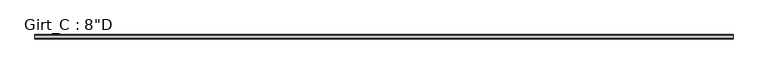
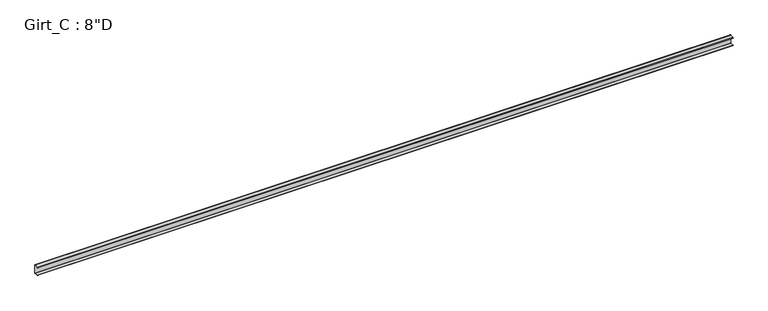
"""IFC4 building model written with IfcOpenShell, lengths in millimetres: beam geometry."""

from ifc_helpers import new_model, si_unit, point, frame, frame_2d, origin, place, context, project, spatial, polyline, circle_curve, trimmed, segment, composite_curve, outline, extrude, source, transform, mapped, element, save


def beam_ff75d66e(model_context):
    return source(origin(), model_context, "Body", "SweptSolid", [
        extrude(outline(composite_curve([segment(polyline([(-87.5109375, 101.6), (-3.3734375, 101.6)]), True, "CONTINUOUS"), segment(trimmed(circle_curve(frame_2d((-3.3734375, 96.8375)), 4.7625), [point((-3.3734375, 101.6))], [point((1.3890625, 96.8375))], False, "CARTESIAN"), True, "CONTINUOUS"), segment(polyline([(1.3890625, 96.8375), (1.3890625, -96.8375)]), True, "CONTINUOUS"), segment(trimmed(circle_curve(frame_2d((-3.3734375, -96.8375)), 4.7625), [point((1.3890625, -96.8375))], [point((-3.3734375, -101.6))], False, "CARTESIAN"), True, "CONTINUOUS"), segment(polyline([(-3.3734375, -101.6), (-87.5109375, -101.6), (-99.7792647, -86.979177), (-97.6510975, -85.1934327), (-86.2154765, -98.821875), (-3.2694106, -98.821875)]), True, "CONTINUOUS"), segment(trimmed(circle_curve(frame_2d((-3.3748024, -96.8389339)), 1.9857399), [point((-3.2694106, -98.821875))], [point((-1.3890625, -96.8389339))], True, "CARTESIAN"), True, "CONTINUOUS"), segment(polyline([(-1.3890625, -96.8389339), (-1.3890625, 96.8381931)]), True, "CONTINUOUS"), segment(trimmed(circle_curve(frame_2d((-3.3741066, 96.8381931)), 1.9850441), [point((-1.3890625, 96.8381931))], [point((-3.3005807, 98.821875))], True, "CARTESIAN"), True, "CONTINUOUS"), segment(polyline([(-3.3005807, 98.821875), (-86.2154765, 98.821875), (-97.6278742, 85.221109), (-99.7560415, 87.0068534), (-87.5109375, 101.6)]), True, "CONTINUOUS")], self_intersect=False)), frame((-7957.5904341, 0.0, 0.0), z_axis=(1.0, 0.0, 0.0), x_axis=(0.0, 1.0, 0.0)), (0.0, 0.0, 1.0), 15851.7537415),
    ])


if __name__ == "__main__":
    model = new_model("IFC4")
    model_context = context("Model", 3, world=origin())
    ifc_project = project(units=[si_unit("LENGTHUNIT", "METRE", prefix="MILLI")], contexts=[model_context])
    site = spatial("IfcSite", under=ifc_project)
    building = spatial("IfcBuilding", under=site)
    placement = place(None, origin())
    beam_shape = beam_ff75d66e(model_context)
    element("IfcBeam", 1, ObjectType="Girt_C : 8\"D", at=placement, inside=building, context=model_context, shape_type="MappedRepresentation", body=[
        mapped(beam_shape, transform((0.0, 0.0, 0.0), x_axis=(1.0, 0.0, 0.0), y_axis=(0.0, 1.0, 0.0), z_axis=(0.0, 0.0, 1.0))),
    ])
    save(model, "model.ifc")

# Revit data of these elements
# Type "Girt_C : 8\"D"
#   half leg = 0' - 1 3/4"
#   Web_Thickness = 0' - 0 7/64"
#   Length [instance default] = 10' - 0"
#   Leg_1 = 0' - 3 1/2"
#   Height = 0' - 8"
#   Structural Material [instance default] = none
# Element 1 (IfcBeam, "Girt_C : 8\"D")
#   Structural Material = GALVANIZED 'CEE' SECTION (8.0x3.5C - SEE STRUCT. DWGS)
#   Materials on its faces: "GALVANIZED 'CEE' SECTION (8.0x3.5C - SEE STRUCT. DWGS)"
# Materials
#   "GALVANIZED 'CEE' SECTION (8.0x3.5C - SEE STRUCT. DWGS)": class "Metal", colour RGB 137 146 153, transparency 0, Description = "Steel, mill finish", Cost = 0
